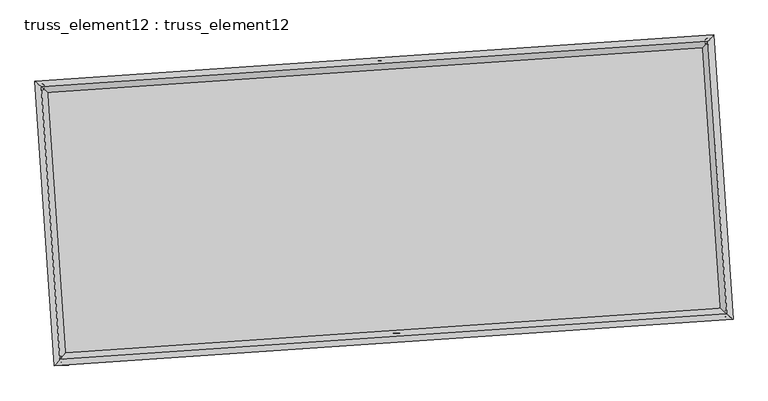
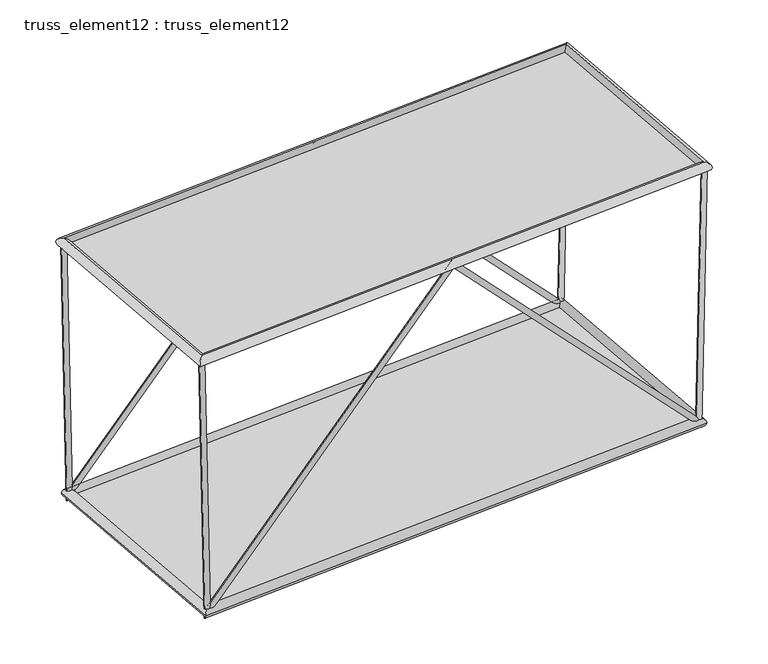
"""IFC4 building model written with IfcOpenShell, lengths in millimetres: plate geometry, truss_element12 : truss_element12."""

from ifc_helpers import new_model, si_unit, frame, origin, origin_with_axes, place, context, project, spatial, polyline, circle_curve, ellipse_curve, outline, extrude, source, transform, mapped, element, save
from ifc_brep_helpers import plane_surface, cylinder_surface, advanced_brep


def truss_element12_truss_element12_76994cec(model_context):
    return source(origin(), model_context, "Body", "SolidModel", [
        advanced_brep(
        [(-3772.049998, 2268.9206632, 4999.9186848), (-3871.1304173, 2255.5609742, 4997.7764407), (-3667.5330566, 2276.0472761, 121.4869998), (-3761.4538263, 2263.039404, -121.4869998), (1063.1340796, 2598.6134851, 5070.9753809), (1063.5910215, 2592.0408705, 4926.7446185), (5794.9440665, 2921.2576209, 121.4949695), (5889.8169105, 2921.1228676, -121.4949695), (5898.3266493, 2928.3068862, 4999.9319376), (5998.3039683, 2928.5201877, 4997.8129357)],
        [
            (0, 1, circle_curve(frame((-3821.5902076, 2262.2408187, 4998.8475628), z_axis=(-0.021419353246380224, -0.0014605042752863, 0.9997695125546531), x_axis=(-0.13359738475228145, 0.9910346805328972, -0.0014144852100089341)), 50.0)),
            (1, 0, circle_curve(frame((-3821.5902076, 2262.2408187, 4998.8475628), z_axis=(-0.021419353246380224, -0.0014605042752863, 0.9997695125546531), x_axis=(-0.13359738475228145, 0.9910346805328972, -0.0014144852100089341)), 50.0)),
            (0, 2),
            (2, 3, ellipse_curve(frame((-3714.4934414, 2269.54334, 0.0), z_axis=(-0.9297185901459638, -0.06339397647082473, 0.36277340983624734), x_axis=(0.36193300753109026, 0.02467883594737901, 0.9318773809443934)), 130.6518852, 50.0)),
            (3, 1),
            (3, 2, ellipse_curve(frame((-3714.4934414, 2269.54334, 0.0), z_axis=(-0.9297185901459638, -0.06339397647082473, 0.36277340983624734), x_axis=(0.36193300753109026, 0.02467883594737901, 0.9318773809443934)), 130.6518852, 50.0)),
            (2, 4),
            (4, 5, ellipse_curve(frame((1063.3625506, 2595.3271778, 4998.8599997), z_axis=(-0.9976833942347468, -0.06802823810323122, -6.073553142254104e-05), x_axis=(6.059483125202198e-05, 4.131731200550759e-06, -0.9999999981555978)), 72.2724119, 50.0)),
            (5, 3),
            (5, 4, ellipse_curve(frame((1063.3625506, 2595.3271778, 4998.8599997), z_axis=(-0.9976833942347468, -0.06802823810323122, -6.073553142254104e-05), x_axis=(6.059483125202198e-05, 4.131731200550759e-06, -0.9999999981555978)), 72.2724119, 50.0)),
            (4, 6),
            (6, 7, ellipse_curve(frame((5842.3804885, 2921.1902443, 0.0), z_axis=(-0.9296544314303244, -0.0633896017318953, -0.3629385574918042), x_axis=(-0.36209777260494025, -0.02469007065143419, 0.9318130732533045)), 130.6694735, 50.0)),
            (7, 5),
            (7, 6, ellipse_curve(frame((5842.3804885, 2921.1902443, 0.0), z_axis=(-0.9296544314303244, -0.0633896017318953, -0.3629385574918042), x_axis=(-0.36209777260494025, -0.02469007065143419, 0.9318130732533045)), 130.6694735, 50.0)),
            (8, 9, circle_curve(frame((5948.3153088, 2928.413537, 4998.8724366), z_axis=(0.0211869640598208, 0.0014446585400487446, 0.9997744873298331), x_axis=(-0.002163146689853894, 0.9999966815980605, -0.0013991387584343373)), 50.0)),
            (9, 8, circle_curve(frame((5948.3153088, 2928.413537, 4998.8724366), z_axis=(0.0211869640598208, 0.0014446585400487446, 0.9997744873298331), x_axis=(-0.002163146689853894, 0.9999966815980605, -0.0013991387584343373)), 50.0)),
            (6, 8),
            (9, 7),
        ],
        [
            plane_surface(frame((-3821.5902076, 2312.2407653, 4998.9206047), z_axis=(-0.021419353246380946, -0.0014605042752824442, 0.9997695125546533), x_axis=(0.999770579336333, -3.129023561676546e-05, 0.02141933039136389))),
            cylinder_surface(frame((-3821.5902076, 2262.2408187, 4998.8475628), z_axis=(-0.021419353246380227, -0.0014605042752863003, 0.9997695125546533), x_axis=(-0.13359738475228145, 0.9910346805328972, -0.0014144852100089341)), 50.0),
            cylinder_surface(frame((-3714.4934414, 2269.54334, 0.0), z_axis=(-0.690180474647465, -0.047060782944605695, -0.7221053905933958), x_axis=(-0.02041492117700933, 0.9987521624772716, -0.045577943572632514)), 50.0),
            cylinder_surface(frame((1063.3625506, 2595.3271778, 4998.8599997), z_axis=(-0.690267981264, -0.04706674968814342, 0.7220213536423394), x_axis=(-0.11534041334180443, 0.9922795540121321, -0.04558372230990076)), 50.0),
            plane_surface(frame((5948.3153088, 2878.4135892, 4998.9446858), z_axis=(0.021186964059822382, 0.0014446585400489178, 0.9997744873298331), x_axis=(0.9997755310838168, -3.061480063770717e-05, -0.021186941940879226))),
            cylinder_surface(frame((5842.3804885, 2921.1902443, 0.0), z_axis=(-0.0211869640598208, -0.0014446585400487446, -0.9997744873298331), x_axis=(-0.002163146689853894, 0.9999966815980605, -0.0013991387584343373)), 50.0),
        ],
        [
            (0, [[1, 2]]),
            (1, [[-1, 3, 4, 5]]),
            (1, [[-2, -5, 6, -3]]),
            (2, [[-4, 7, 8, 9]]),
            (2, [[-6, -9, 10, -7]]),
            (3, [[-8, 11, 12, 13]]),
            (3, [[-10, -13, 14, -11]]),
            (4, [[15, 16]]),
            (5, [[-12, 17, -16, 18]]),
            (5, [[-14, -18, -15, -17]]),
        ],
    ),
        advanced_brep(
        [(-3499.9370451, -1721.8129211, 4999.9186848), (-3599.0174644, -1735.1726101, 4997.7764407), (-3395.4201037, -1714.6863082, 121.4869998), (-3489.3408733, -1727.6941803, -121.4869998), (1335.2470325, -1392.1200992, 5070.9753809), (1335.7039744, -1398.6927138, 4926.7446185), (6067.0570194, -1069.4759634, 121.4949695), (6161.9298635, -1069.6107167, -121.4949695), (6170.4396022, -1062.4266981, 4999.9319376), (6270.4169213, -1062.2133966, 4997.8129357)],
        [
            (0, 1, circle_curve(frame((-3549.4772547, -1728.4927656, 4998.8475628), z_axis=(-0.021419353246380154, -0.0014605042752862817, 0.9997695125546531), x_axis=(-0.13359738475228128, 0.9910346805328972, -0.00141448521000894)), 50.0)),
            (1, 0, circle_curve(frame((-3549.4772547, -1728.4927656, 4998.8475628), z_axis=(-0.021419353246380154, -0.0014605042752862817, 0.9997695125546531), x_axis=(-0.13359738475228128, 0.9910346805328972, -0.00141448521000894)), 50.0)),
            (0, 2),
            (2, 3, ellipse_curve(frame((-3442.3804885, -1721.1902443, 0.0), z_axis=(-0.9297185901459636, -0.0633939764708246, 0.36277340983624784), x_axis=(0.36193300753109076, 0.02467883594737902, 0.9318773809443933)), 130.6518852, 50.0)),
            (3, 1),
            (3, 2, ellipse_curve(frame((-3442.3804885, -1721.1902443, 0.0), z_axis=(-0.9297185901459636, -0.0633939764708246, 0.36277340983624784), x_axis=(0.36193300753109076, 0.02467883594737902, 0.9318773809443933)), 130.6518852, 50.0)),
            (2, 4),
            (4, 5, ellipse_curve(frame((1335.4755035, -1395.4064065, 4998.8599997), z_axis=(-0.9976833942347468, -0.0680282381032311, -6.073553142181889e-05), x_axis=(6.059483125125319e-05, 4.1317312004738805e-06, -0.9999999981555978)), 72.2724119, 50.0)),
            (5, 3),
            (5, 4, ellipse_curve(frame((1335.4755035, -1395.4064065, 4998.8599997), z_axis=(-0.9976833942347468, -0.0680282381032311, -6.073553142181889e-05), x_axis=(6.059483125125319e-05, 4.1317312004738805e-06, -0.9999999981555978)), 72.2724119, 50.0)),
            (4, 6),
            (6, 7, ellipse_curve(frame((6114.4934414, -1069.54334, 0.0), z_axis=(-0.9296544314303247, -0.06338960173189526, -0.36293855749180376), x_axis=(-0.36209777260493975, -0.02469007065143407, 0.9318130732533046)), 130.6694735, 50.0)),
            (7, 5),
            (7, 6, ellipse_curve(frame((6114.4934414, -1069.54334, 0.0), z_axis=(-0.9296544314303247, -0.06338960173189526, -0.36293855749180376), x_axis=(-0.36209777260493975, -0.02469007065143407, 0.9318130732533046)), 130.6694735, 50.0)),
            (8, 9, circle_curve(frame((6220.4282617, -1062.3200473, 4998.8724366), z_axis=(0.02118696405982117, 0.0014446585400488233, 0.9997744873298331), x_axis=(-0.002163146689853997, 0.9999966815980605, -0.001399138758434413)), 50.0)),
            (9, 8, circle_curve(frame((6220.4282617, -1062.3200473, 4998.8724366), z_axis=(0.02118696405982117, 0.0014446585400488233, 0.9997744873298331), x_axis=(-0.002163146689853997, 0.9999966815980605, -0.001399138758434413)), 50.0)),
            (6, 8),
            (9, 7),
        ],
        [
            plane_surface(frame((-3549.4772547, -1678.492819, 4998.9206047), z_axis=(-0.021419353246380946, -0.0014605042752824403, 0.9997695125546533), x_axis=(0.999770579336333, -3.129023561676546e-05, 0.02141933039136389))),
            cylinder_surface(frame((-3549.4772547, -1728.4927656, 4998.8475628), z_axis=(-0.021419353246380154, -0.0014605042752862817, 0.9997695125546531), x_axis=(-0.13359738475228128, 0.9910346805328972, -0.00141448521000894)), 50.0),
            cylinder_surface(frame((-3442.3804885, -1721.1902443, 0.0), z_axis=(-0.6901804746474656, -0.04706078294460567, -0.7221053905933954), x_axis=(-0.02041492117700938, 0.9987521624772717, -0.04557794357263245)), 50.0),
            cylinder_surface(frame((1335.4755035, -1395.4064065, 4998.8599997), z_axis=(-0.6902679812639996, -0.04706674968814329, 0.7220213536423399), x_axis=(-0.11534041334180421, 0.9922795540121322, -0.045583722309900654)), 50.0),
            plane_surface(frame((6220.4282617, -1112.3199951, 4998.9446858), z_axis=(0.021186964059822382, 0.001444658540048914, 0.9997744873298331), x_axis=(0.9997755310838168, -3.061480063770717e-05, -0.021186941940879226))),
            cylinder_surface(frame((6114.4934414, -1069.54334, 0.0), z_axis=(-0.02118696405982117, -0.0014446585400488233, -0.9997744873298331), x_axis=(-0.002163146689853997, 0.9999966815980605, -0.001399138758434413)), 50.0),
        ],
        [
            (0, [[1, 2]]),
            (1, [[-1, 3, 4, 5]]),
            (1, [[-2, -5, 6, -3]]),
            (2, [[-4, 7, 8, 9]]),
            (2, [[-6, -9, 10, -7]]),
            (3, [[-8, 11, 12, 13]]),
            (3, [[-10, -13, 14, -11]]),
            (4, [[15, 16]]),
            (5, [[-12, 17, -16, 18]]),
            (5, [[-14, -18, -15, -17]]),
        ],
    ),
        advanced_brep(
        [(-3549.4707858, -1728.4855958, 4908.847563), (-3549.4837237, -1728.4999355, 5088.8475625), (-3821.59759, 2262.247044, 5088.8475625), (-3821.5828253, 2262.2345933, 4908.847563), (5948.3213216, 2928.4206757, 5088.8724364), (5948.309296, 2928.4063982, 4908.8724369), (6220.4351879, -1062.3263038, 5088.8724364), (6220.4213355, -1062.3137909, 4908.8724369)],
        [
            (0, 1, ellipse_curve(frame((-3549.4772547, -1728.4927656, 4998.8475628), z_axis=(-0.7535719234031822, 0.6573654662782359, -1.7961013785196693e-06), x_axis=(-0.6573654662758049, -0.7535719234053027, -1.796101378519747e-06)), 127.2792206, 90.0)),
            (1, 2),
            (2, 3, ellipse_curve(frame((-3821.5902076, 2262.2408187, 4998.8475628), z_axis=(-0.6573654662758047, -0.753571923405303, -1.7961013785198175e-06), x_axis=(0.7535719234031824, -0.6573654662782357, 1.7961013785197407e-06)), 127.2792206, 90.0)),
            (3, 0),
            (1, 0, ellipse_curve(frame((-3549.4772547, -1728.4927656, 4998.8475628), z_axis=(-0.7535719234031822, 0.6573654662782359, -1.7961013785196693e-06), x_axis=(-0.6573654662758049, -0.7535719234053027, -1.796101378519747e-06)), 127.2792206, 90.0)),
            (3, 2, ellipse_curve(frame((-3821.5902076, 2262.2408187, 4998.8475628), z_axis=(-0.6573654662758047, -0.753571923405303, -1.7961013785198175e-06), x_axis=(0.7535719234031824, -0.6573654662782357, 1.7961013785197407e-06)), 127.2792206, 90.0)),
            (2, 4),
            (4, 5, ellipse_curve(frame((5948.3153088, 2928.413537, 4998.8724366), z_axis=(-0.7535719234031821, 0.657365466278236, -1.7961013785198129e-06), x_axis=(-0.6573654662758048, -0.7535719234053028, -1.7961013785197449e-06)), 127.2792206, 90.0)),
            (5, 3),
            (5, 4, ellipse_curve(frame((5948.3153088, 2928.413537, 4998.8724366), z_axis=(-0.7535719234031821, 0.657365466278236, -1.7961013785198129e-06), x_axis=(-0.6573654662758048, -0.7535719234053028, -1.7961013785197449e-06)), 127.2792206, 90.0)),
            (4, 6),
            (6, 7, ellipse_curve(frame((6220.4282617, -1062.3200473, 4998.8724366), z_axis=(0.6573654662758048, 0.7535719234053028, 1.7961013785196735e-06), x_axis=(-0.7535719234031819, 0.6573654662782361, -1.7961013785197413e-06)), 127.2792206, 90.0)),
            (7, 5),
            (7, 6, ellipse_curve(frame((6220.4282617, -1062.3200473, 4998.8724366), z_axis=(0.6573654662758048, 0.7535719234053028, 1.7961013785196735e-06), x_axis=(-0.7535719234031819, 0.6573654662782361, -1.7961013785197413e-06)), 127.2792206, 90.0)),
            (6, 1),
            (0, 7),
        ],
        [
            cylinder_surface(frame((-3549.4772547, -1728.4927656, 4998.8475628), z_axis=(0.0680282382287017, -0.9976833960748767, 0.0), x_axis=(-0.9976833931072081, -0.06802823802634766, -7.713052989256367e-05)), 90.0),
            cylinder_surface(frame((-3821.5902076, 2262.2408187, 4998.8475628), z_axis=(-0.9976833960716581, -0.06802823822848202, -2.5400709288996837e-06), x_axis=(-0.06802823785042973, 0.9976833933123418, -7.459045897073017e-05)), 90.0),
            cylinder_surface(frame((5948.3153088, 2928.413537, 4998.8724366), z_axis=(-0.06802823822870112, 0.9976833960748768, 0.0), x_axis=(0.9976833934852605, 0.06802823805212503, -7.205038804889673e-05)), 90.0),
            cylinder_surface(frame((6220.4282617, -1062.3200473, 4998.8724366), z_axis=(0.9976833960716582, 0.06802823822848199, 2.5400709288995833e-06), x_axis=(0.06802823822848199, -0.9976833932865639, -7.459045897073023e-05)), 90.0),
        ],
        [
            (0, [[1, 2, 3, 4]]),
            (0, [[5, -4, 6, -2]]),
            (1, [[-3, 7, 8, 9]]),
            (1, [[-6, -9, 10, -7]]),
            (2, [[-8, 11, 12, 13]]),
            (2, [[-10, -13, 14, -11]]),
            (3, [[-12, 15, -1, 16]]),
            (3, [[-14, -16, -5, -15]]),
        ],
    ),
        advanced_brep(
        [(-3358.7115243, -1625.2761972, 0.0), (-3526.0494527, -1817.1042913, 0.0), (-3810.4074885, 2353.2123043, 0.0), (-3618.5793943, 2185.8743758, 0.0), (5926.0494527, 3017.1042913, 0.0), (5758.7115243, 2825.2761972, 0.0), (6210.4074885, -1153.2123043, 0.0), (6018.5793943, -985.8743758, 0.0)],
        [
            (0, 1, ellipse_curve(frame((-3442.3804885, -1721.1902443, 0.0), z_axis=(-0.753571923405459, 0.6573654662780797, 0.0), x_axis=(-0.6573654662780797, -0.7535719234054589, 0.0)), 127.2792206, 90.0)),
            (1, 2),
            (2, 3, ellipse_curve(frame((-3714.4934414, 2269.54334, 0.0), z_axis=(-0.6573654662780796, -0.7535719234054591, 0.0), x_axis=(0.753571923405459, -0.6573654662780795, 0.0)), 127.2792206, 90.0)),
            (3, 0),
            (1, 0, ellipse_curve(frame((-3442.3804885, -1721.1902443, 0.0), z_axis=(-0.753571923405459, 0.6573654662780797, 0.0), x_axis=(-0.6573654662780797, -0.7535719234054589, 0.0)), 127.2792206, 90.0)),
            (3, 2, ellipse_curve(frame((-3714.4934414, 2269.54334, 0.0), z_axis=(-0.6573654662780796, -0.7535719234054591, 0.0), x_axis=(0.753571923405459, -0.6573654662780795, 0.0)), 127.2792206, 90.0)),
            (2, 4),
            (4, 5, ellipse_curve(frame((5842.3804885, 2921.1902443, 0.0), z_axis=(-0.7535719234054591, 0.6573654662780795, 0.0), x_axis=(-0.6573654662780795, -0.7535719234054591, 0.0)), 127.2792206, 90.0)),
            (5, 3),
            (5, 4, ellipse_curve(frame((5842.3804885, 2921.1902443, 0.0), z_axis=(-0.7535719234054591, 0.6573654662780795, 0.0), x_axis=(-0.6573654662780795, -0.7535719234054591, 0.0)), 127.2792206, 90.0)),
            (4, 6),
            (6, 7, ellipse_curve(frame((6114.4934414, -1069.54334, 0.0), z_axis=(0.6573654662780796, 0.753571923405459, 0.0), x_axis=(-0.753571923405459, 0.6573654662780796, 0.0)), 127.2792206, 90.0)),
            (7, 5),
            (7, 6, ellipse_curve(frame((6114.4934414, -1069.54334, 0.0), z_axis=(0.6573654662780796, 0.753571923405459, 0.0), x_axis=(-0.753571923405459, 0.6573654662780796, 0.0)), 127.2792206, 90.0)),
            (6, 1),
            (0, 7),
        ],
        [
            cylinder_surface(frame((-3442.3804885, -1721.1902443, 0.0), z_axis=(0.06802823822870296, -0.9976833960748764, 0.0), x_axis=(-0.9976833960748764, -0.06802823822870296, 0.0)), 90.0),
            cylinder_surface(frame((-3714.4934414, 2269.54334, 0.0), z_axis=(-0.9976833960748764, -0.06802823822870285, 0.0), x_axis=(-0.06802823822870285, 0.9976833960748764, 0.0)), 90.0),
            cylinder_surface(frame((5842.3804885, 2921.1902443, 0.0), z_axis=(-0.0680282382287031, 0.9976833960748764, 0.0), x_axis=(0.9976833960748764, 0.0680282382287031, 0.0)), 90.0),
            cylinder_surface(frame((6114.4934414, -1069.54334, 0.0), z_axis=(0.9976833960748764, 0.06802823822870266, 0.0), x_axis=(0.06802823822870266, -0.9976833960748764, 0.0)), 90.0),
        ],
        [
            (0, [[1, 2, 3, 4]]),
            (0, [[5, -4, 6, -2]]),
            (1, [[-3, 7, 8, 9]]),
            (1, [[-6, -9, 10, -7]]),
            (2, [[-8, 11, 12, 13]]),
            (2, [[-10, -13, 14, -11]]),
            (3, [[-12, 15, -1, 16]]),
            (3, [[-14, -16, -5, -15]]),
        ],
    ),
        extrude(outline(polyline([(-3442.3804885, -1721.1902443), (-3714.4934414, 2269.54334), (5842.3804885, 2921.1902443), (6114.4934414, -1069.54334), (-3442.3804885, -1721.1902443)])), origin_with_axes(), (0.0, 0.0, 1.0), 20.0),
        extrude(outline(polyline([(-2000.0, 4896.2955356), (2000.0, 4896.2955356), (2000.0, -4896.2955357), (-2000.0, -4896.2955357), (-2000.0, 4896.2955356)])), frame((1199.419027, 599.9603857, 4998.8599997), z_axis=(-2.5341865906156524e-06, -1.7279655026898703e-07, 0.9999999999967741), x_axis=(-0.06802823822870295, 0.9976833960748765, 0.0)), (0.0, 0.0, 1.0), 20.0),
    ])


if __name__ == "__main__":
    model = new_model("IFC4")
    model_context = context("Model", 3, world=origin())
    ifc_project = project(units=[si_unit("LENGTHUNIT", "METRE", prefix="MILLI")], contexts=[model_context])
    site = spatial("IfcSite", under=ifc_project)
    building = spatial("IfcBuilding", under=site)
    placement = place(None, origin())
    truss_element12_truss_element12_shape = truss_element12_truss_element12_76994cec(model_context)
    element("IfcPlate", 1, ObjectType="truss_element12 : truss_element12", at=placement, inside=building, context=model_context, shape_type="MappedRepresentation", body=[
        mapped(truss_element12_truss_element12_shape, transform((0.0, 0.0, 0.0), x_axis=(1.0, 0.0, 0.0), y_axis=(0.0, 1.0, 0.0), z_axis=(0.0, 0.0, 1.0))),
    ])
    save(model, "model.ifc")

# Revit data of these elements
# Type "truss_element12 : truss_element12"
#   steellbar1 = 90 mm
#   steelbar2 = 50 mm
#   offset1 = 5000 mm
#   M = Default Roof
# Element 1 (IfcPlate, "truss_element12 : truss_element12")
#   Materials on its faces: "Default Roof"
# Materials
#   "Default Roof": class "Miscellaneous", colour RGB 0 127 0, transparency 0, Comments = "Rendering appearance not upgraded Rendering appearance not upgraded ", Cost = 0
